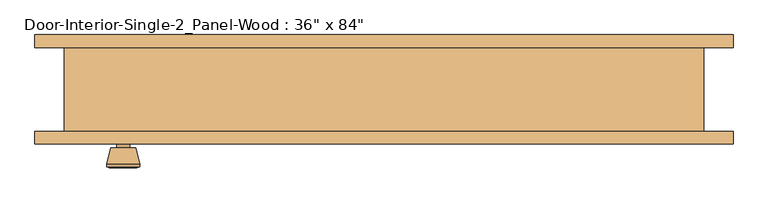
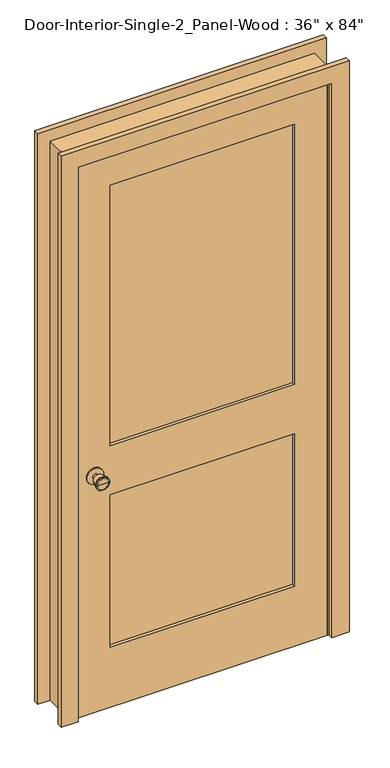
"""IFC4 building model written with IfcOpenShell, lengths in millimetres: door geometry."""

from ifc_helpers import new_model, si_unit, point, frame, frame_2d, origin, place, context, project, spatial, polyline, circle_curve, trimmed, segment, composite_curve, outline, extrude, faceted_brep, source, transform, mapped, element, save
from ifc_brep_helpers import plane_surface, cylinder_surface, revolved_surface, advanced_brep


def door_b46e0f67(model_context):
    return source(origin(), model_context, "Body", "SolidModel", [
        advanced_brep(
        [(-393.7, -19.4, 914.4), (-403.7, -19.4, 914.4), (-383.7, -19.4, 914.4), (-373.2241324, 29.6, 914.4), (-414.1758676, 29.6, 914.4), (-393.7, 29.6, 914.4), (-368.7, 27.7721319, 914.4), (-418.7, 27.7721319, 914.4), (-368.7, 24.3084537, 914.4), (-418.7, 24.3084537, 914.4), (-375.063764, -0.4, 914.4), (-412.336236, -0.4, 914.4), (-383.7, -0.4, 914.4), (-403.7, -0.4, 914.4)],
        [
            (0, 1),
            (1, 2, circle_curve(frame((-393.7, -19.4, 914.4), z_axis=(0.0, -1.0, 0.0), x_axis=(-1.0, 0.0, 0.0)), 10.0)),
            (2, 0),
            (2, 1, circle_curve(frame((-393.7, -19.4, 914.4), z_axis=(0.0, -1.0, 0.0), x_axis=(-1.0, 0.0, 0.0)), 10.0)),
            (3, 4, circle_curve(frame((-393.7, 29.6, 914.4), z_axis=(0.0, 1.0, 0.0), x_axis=(-1.0, 0.0, 0.0)), 20.4758676)),
            (4, 5),
            (5, 3),
            (4, 3, circle_curve(frame((-393.7, 29.6, 914.4), z_axis=(0.0, 1.0, 0.0), x_axis=(-1.0, 0.0, 0.0)), 20.4758676)),
            (6, 7, circle_curve(frame((-393.7, 27.7721319, 914.4), z_axis=(0.0, 1.0, 0.0), x_axis=(-1.0, 0.0, 0.0)), 25.0)),
            (7, 4),
            (3, 6),
            (7, 6, circle_curve(frame((-393.7, 27.7721319, 914.4), z_axis=(0.0, 1.0, 0.0), x_axis=(-1.0, 0.0, 0.0)), 25.0)),
            (8, 9, circle_curve(frame((-393.7, 24.3084537, 914.4), z_axis=(0.0, 1.0, 0.0), x_axis=(-1.0, 0.0, 0.0)), 25.0)),
            (9, 7),
            (6, 8),
            (9, 8, circle_curve(frame((-393.7, 24.3084537, 914.4), z_axis=(0.0, 1.0, 0.0), x_axis=(-1.0, 0.0, 0.0)), 25.0)),
            (10, 11, circle_curve(frame((-393.7, -0.4, 914.4), z_axis=(0.0, 1.0, 0.0), x_axis=(-1.0, 0.0, 0.0)), 18.636236)),
            (11, 9),
            (8, 10),
            (11, 10, circle_curve(frame((-393.7, -0.4, 914.4), z_axis=(0.0, 1.0, 0.0), x_axis=(-1.0, 0.0, 0.0)), 18.636236)),
            (12, 13, circle_curve(frame((-393.7, -0.4, 914.4), z_axis=(0.0, 1.0, 0.0), x_axis=(-1.0, 0.0, 0.0)), 10.0)),
            (13, 11),
            (10, 12),
            (13, 12, circle_curve(frame((-393.7, -0.4, 914.4), z_axis=(0.0, 1.0, 0.0), x_axis=(-1.0, 0.0, 0.0)), 10.0)),
            (1, 13),
            (12, 2),
        ],
        [
            plane_surface(frame((-393.7, -19.4, 914.4), z_axis=(0.0, -1.0, 0.0), x_axis=(-1.0, 0.0, 0.0))),
            plane_surface(frame((-393.7, 29.6, 914.4), z_axis=(0.0, 1.0, 0.0), x_axis=(-1.0, 0.0, 0.0))),
            revolved_surface(polyline([(-414.1758676, 29.6, 914.4), (-418.7, 27.7721319, 914.4)]), (-393.7, -19.4, 914.4), (0.0, -1.0, 0.0)),
            cylinder_surface(frame((-393.7, -19.4, 914.4), z_axis=(0.0, -1.0, 0.0), x_axis=(-1.0, 0.0, 0.0)), 25.0),
            revolved_surface(polyline([(-418.7, 24.3084537, 914.4), (-412.336236, -0.4, 914.4)]), (-393.7, -19.4, 914.4), (0.0, -1.0, 0.0)),
            plane_surface(frame((-393.7, -0.4, 914.4), z_axis=(0.0, -1.0, 0.0), x_axis=(-1.0, 0.0, 0.0))),
            cylinder_surface(frame((-393.7, -19.4, 914.4), z_axis=(0.0, -1.0, 0.0), x_axis=(-1.0, 0.0, 0.0)), 10.0),
        ],
        [
            (0, [[1, 2, 3]]),
            (0, [[-3, 4, -1]]),
            (1, [[5, 6, 7]]),
            (1, [[8, -7, -6]]),
            (2, [[9, 10, -5, 11]]),
            (2, [[12, -11, -8, -10]]),
            (3, [[13, 14, -9, 15]]),
            (3, [[16, -15, -12, -14]]),
            (4, [[17, 18, -13, 19]]),
            (4, [[20, -19, -16, -18]]),
            (5, [[21, 22, -17, 23]]),
            (5, [[24, -23, -20, -22]]),
            (6, [[-2, 25, -21, 26]]),
            (6, [[-4, -26, -24, -25]]),
        ],
    ),
        extrude(outline(composite_curve([segment(trimmed(circle_curve(frame_2d((914.4, -393.7)), 30.0), [point((914.4, -423.7))], [point((914.4, -363.7))], False, "CARTESIAN"), True, "CONTINUOUS"), segment(trimmed(circle_curve(frame_2d((914.4, -393.7)), 30.0), [point((914.4, -363.7))], [point((914.4, -423.7))], False, "CARTESIAN"), True, "CONTINUOUS")], self_intersect=False)), frame((0.0, -25.4, 0.0), z_axis=(0.0, 1.0, 0.0), x_axis=(0.0, 0.0, 1.0)), (0.0, 0.0, 1.0), 6.0),
        advanced_brep(
        [(-393.7, -66.325, 914.4), (-383.7, -66.325, 914.4), (-403.7, -66.325, 914.4), (-373.2241324, -115.325, 914.4), (-393.7, -115.325, 914.4), (-414.1758676, -115.325, 914.4), (-368.7, -113.4971319, 914.4), (-418.7, -113.4971319, 914.4), (-368.7, -110.0334537, 914.4), (-418.7, -110.0334537, 914.4), (-375.063764, -85.325, 914.4), (-412.336236, -85.325, 914.4), (-383.7, -85.325, 914.4), (-403.7, -85.325, 914.4)],
        [
            (0, 1),
            (1, 2, circle_curve(frame((-393.7, -66.325, 914.4), z_axis=(0.0, 1.0, 0.0), x_axis=(-1.0, 0.0, 0.0)), 10.0)),
            (2, 0),
            (2, 1, circle_curve(frame((-393.7, -66.325, 914.4), z_axis=(0.0, 1.0, 0.0), x_axis=(-1.0, 0.0, 0.0)), 10.0)),
            (3, 4),
            (4, 5),
            (5, 3, circle_curve(frame((-393.7, -115.325, 914.4), z_axis=(0.0, -1.0, 0.0), x_axis=(-1.0, 0.0, 0.0)), 20.4758676)),
            (3, 5, circle_curve(frame((-393.7, -115.325, 914.4), z_axis=(0.0, -1.0, 0.0), x_axis=(-1.0, 0.0, 0.0)), 20.4758676)),
            (6, 3),
            (5, 7),
            (7, 6, circle_curve(frame((-393.7, -113.4971319, 914.4), z_axis=(0.0, -1.0, 0.0), x_axis=(-1.0, 0.0, 0.0)), 25.0)),
            (6, 7, circle_curve(frame((-393.7, -113.4971319, 914.4), z_axis=(0.0, -1.0, 0.0), x_axis=(-1.0, 0.0, 0.0)), 25.0)),
            (8, 6),
            (7, 9),
            (9, 8, circle_curve(frame((-393.7, -110.0334537, 914.4), z_axis=(0.0, -1.0, 0.0), x_axis=(-1.0, 0.0, 0.0)), 25.0)),
            (8, 9, circle_curve(frame((-393.7, -110.0334537, 914.4), z_axis=(0.0, -1.0, 0.0), x_axis=(-1.0, 0.0, 0.0)), 25.0)),
            (10, 8),
            (9, 11),
            (11, 10, circle_curve(frame((-393.7, -85.325, 914.4), z_axis=(0.0, -1.0, 0.0), x_axis=(-1.0, 0.0, 0.0)), 18.636236)),
            (10, 11, circle_curve(frame((-393.7, -85.325, 914.4), z_axis=(0.0, -1.0, 0.0), x_axis=(-1.0, 0.0, 0.0)), 18.636236)),
            (12, 10),
            (11, 13),
            (13, 12, circle_curve(frame((-393.7, -85.325, 914.4), z_axis=(0.0, -1.0, 0.0), x_axis=(-1.0, 0.0, 0.0)), 10.0)),
            (12, 13, circle_curve(frame((-393.7, -85.325, 914.4), z_axis=(0.0, -1.0, 0.0), x_axis=(-1.0, 0.0, 0.0)), 10.0)),
            (1, 12),
            (13, 2),
        ],
        [
            plane_surface(frame((-393.7, -66.325, 914.4), z_axis=(0.0, 1.0, 0.0), x_axis=(-1.0, 0.0, 0.0))),
            plane_surface(frame((-393.7, -115.325, 914.4), z_axis=(0.0, -1.0, 0.0), x_axis=(-1.0, 0.0, 0.0))),
            revolved_surface(polyline([(-414.1758676, -115.325, 914.4), (-418.7, -113.4971319, 914.4)]), (-393.7, -66.325, 914.4), (0.0, 1.0, 0.0)),
            cylinder_surface(frame((-393.7, -66.325, 914.4), z_axis=(0.0, 1.0, 0.0), x_axis=(-1.0, 0.0, 0.0)), 25.0),
            revolved_surface(polyline([(-418.7, -110.0334537, 914.4), (-412.336236, -85.325, 914.4)]), (-393.7, -66.325, 914.4), (0.0, 1.0, 0.0)),
            plane_surface(frame((-393.7, -85.325, 914.4), z_axis=(0.0, 1.0, 0.0), x_axis=(-1.0, 0.0, 0.0))),
            cylinder_surface(frame((-393.7, -66.325, 914.4), z_axis=(0.0, 1.0, 0.0), x_axis=(-1.0, 0.0, 0.0)), 10.0),
        ],
        [
            (0, [[1, 2, 3]]),
            (0, [[-3, 4, -1]]),
            (1, [[5, 6, 7]]),
            (1, [[-6, -5, 8]]),
            (2, [[9, -7, 10, 11]]),
            (2, [[-10, -8, -9, 12]]),
            (3, [[13, -11, 14, 15]]),
            (3, [[-14, -12, -13, 16]]),
            (4, [[17, -15, 18, 19]]),
            (4, [[-18, -16, -17, 20]]),
            (5, [[21, -19, 22, 23]]),
            (5, [[-22, -20, -21, 24]]),
            (6, [[25, -23, 26, -2]]),
            (6, [[-26, -24, -25, -4]]),
        ],
    ),
        extrude(outline(composite_curve([segment(trimmed(circle_curve(frame_2d((914.4, -393.7)), 30.0), [point((914.4, -423.7))], [point((914.4, -363.7))], False, "CARTESIAN"), True, "CONTINUOUS"), segment(trimmed(circle_curve(frame_2d((914.4, -393.7)), 30.0), [point((914.4, -363.7))], [point((914.4, -423.7))], False, "CARTESIAN"), True, "CONTINUOUS")], self_intersect=False)), frame((0.0, -66.325, 0.0), z_axis=(0.0, 1.0, 0.0), x_axis=(0.0, 0.0, 1.0)), (0.0, 0.0, 1.0), 6.0),
        extrude(outline(polyline([(336.55, -37.0416667), (336.55, -48.6833333), (-336.55, -48.6833333), (-336.55, -37.0416667), (336.55, -37.0416667)])), frame((0.0, 0.0, 1009.65), z_axis=(0.0, 0.0, 1.0), x_axis=(1.0, 0.0, 0.0)), (0.0, 0.0, 1.0), 1004.8875),
        extrude(outline(polyline([(336.55, -37.0416667), (336.55, -48.6833333), (-336.55, -48.6833333), (-336.55, -37.0416667), (336.55, -37.0416667)])), frame((0.0, 0.0, 231.775), z_axis=(0.0, 0.0, 1.0), x_axis=(1.0, 0.0, 0.0)), (0.0, 0.0, 1.0), 587.375),
        extrude(outline(polyline([(2133.6, -457.2), (0.0, -457.2), (0.0, 457.2), (2133.6, 457.2), (2133.6, -457.2)]), holes=[polyline([(2014.5375, -336.55), (2014.5375, 336.55), (1009.65, 336.55), (1009.65, -336.55), (2014.5375, -336.55)]), polyline([(819.15, -336.55), (819.15, 336.55), (231.775, 336.55), (231.775, -336.55), (819.15, -336.55)])]), frame((0.0, -60.325, 0.0), z_axis=(0.0, 1.0, 0.0), x_axis=(0.0, 0.0, 1.0)), (0.0, 0.0, 1.0), 34.925),
        faceted_brep([(482.6, -60.325, 0.0), (457.2, -60.325, 0.0), (457.2, -25.4, 0.0), (444.5, -25.4, 0.0), (444.5, 9.525, 0.0), (457.2, 9.525, 0.0), (457.2, 66.675, 0.0), (482.6, 66.675, 0.0), (482.6, 66.675, 2159.0), (482.6, -60.325, 2159.0), (457.2, 66.675, 2133.6), (-457.2, 66.675, 2133.6), (-457.2, 66.675, 0.0), (-482.6, 66.675, 0.0), (-482.6, 66.675, 2159.0), (457.2, 9.525, 2133.6), (444.5, 9.525, 2120.9), (-444.5, 9.525, 2120.9), (-444.5, 9.525, 0.0), (-457.2, 9.525, 0.0), (-457.2, 9.525, 2133.6), (444.5, -25.4, 2120.9), (457.2, -25.4, 2133.6), (-457.2, -25.4, 2133.6), (-457.2, -25.4, 0.0), (-444.5, -25.4, 0.0), (-444.5, -25.4, 2120.9), (457.2, -60.325, 2133.6), (-482.6, -60.325, 2159.0), (-482.6, -60.325, 0.0), (-457.2, -60.325, 0.0), (-457.2, -60.325, 2133.6)], [[[0, 1, 2, 3, 4, 5, 6, 7]], [[7, 8, 9, 0]], [[6, 10, 11, 12, 13, 14, 8, 7]], [[5, 15, 10, 6]], [[4, 16, 17, 18, 19, 20, 15, 5]], [[3, 21, 16, 4]], [[2, 22, 23, 24, 25, 26, 21, 3]], [[1, 27, 22, 2]], [[0, 9, 28, 29, 30, 31, 27, 1]], [[8, 14, 28, 9]], [[15, 20, 11, 10]], [[21, 26, 17, 16]], [[27, 31, 23, 22]], [[29, 13, 12, 19, 18, 25, 24, 30]], [[14, 13, 29, 28]], [[20, 19, 12, 11]], [[26, 25, 18, 17]], [[31, 30, 24, 23]]]),
        extrude(outline(polyline([(0.0, 527.05), (2203.45, 527.05), (2203.45, -527.05), (0.0, -527.05), (0.0, -463.55), (2139.95, -463.55), (2139.95, 463.55), (0.0, 463.55), (0.0, 527.05)])), frame((0.0, 66.675, 0.0), z_axis=(0.0, 1.0, 0.0), x_axis=(0.0, 0.0, 1.0)), (0.0, 0.0, 1.0), 19.05),
        extrude(outline(polyline([(0.0, 527.05), (2203.45, 527.05), (2203.45, -527.05), (0.0, -527.05), (0.0, -463.55), (2139.95, -463.55), (2139.95, 463.55), (0.0, 463.55), (0.0, 527.05)])), frame((0.0, -79.375, 0.0), z_axis=(0.0, 1.0, 0.0), x_axis=(0.0, 0.0, 1.0)), (0.0, 0.0, 1.0), 19.05),
    ])


if __name__ == "__main__":
    model = new_model("IFC4")
    model_context = context("Model", 3, world=origin())
    ifc_project = project(units=[si_unit("LENGTHUNIT", "METRE", prefix="MILLI")], contexts=[model_context])
    site = spatial("IfcSite", under=ifc_project)
    building = spatial("IfcBuilding", under=site)
    placement = place(None, origin())
    door_shape = door_b46e0f67(model_context)
    element("IfcDoor", 1, ObjectType="Door-Interior-Single-2_Panel-Wood : 36\" x 84\"", at=placement, inside=building, context=model_context, shape_type="MappedRepresentation", body=[
        mapped(door_shape, transform((0.0, 0.0, 0.0), x_axis=(1.0, 0.0, 0.0), y_axis=(0.0, 1.0, 0.0), z_axis=(0.0, 0.0, 1.0))),
    ])
    save(model, "model.ifc")

# Revit data of these elements
# Type "Door-Interior-Single-2_Panel-Wood : 36\" x 84\""
#   Type Mark = "17"
#   Assembly Code = "C1020300"
#   Analytic Construction = "Wooden"
#   Top Rail = 0' - 4 11/16"
#   Thickness = 0' - 1 3/8"
#   Thermal Resistance (R) = 2.5876 (h·ft²·°F)/BTU
#   Swing Angle [instance default] = 90.00°
#   Stiles = 0' - 4 3/4"
#   Rough Width = 3' - 2"
#   Rough Height = 7' - 1"
#   Lock Rail = 0' - 7 1/2"
#   Height = 7' - 0"
#   Width = 3' - 0"
#   Heat Transfer Coefficient (U) = 0.3865 BTU/(h·ft²·°F)
#   Bottom Rail = 0' - 9 1/8"
#   Function = 0
#   Define Thermal Properties by = 1
#   Trim Material = Cherry
#   Panel Material = Cherry
#   Frame Material = Cherry
#   Door Handle Material = Aluminum
#   Visual Light Transmittance = 0
#   Solar Heat Gain Coefficient = 0
#   Wall Closure = (empty or 0)
#   Function = (empty or 0)
# Element 1 (IfcDoor, "Door-Interior-Single-2_Panel-Wood : 36\" x 84\"")
#   Materials on its faces: "Cherry", "Aluminum"
# Materials
#   "Cherry": class "Wood", colour RGB 157 77 38, transparency 0, Description = "Prunus Serotina", Cost = 0
#   "Aluminum": class "Metal", colour RGB 120 120 120, transparency 0, Description = "Aluminum 6061", Cost = 0
